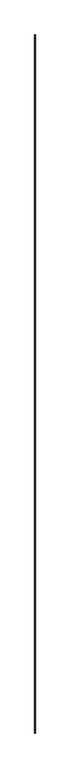
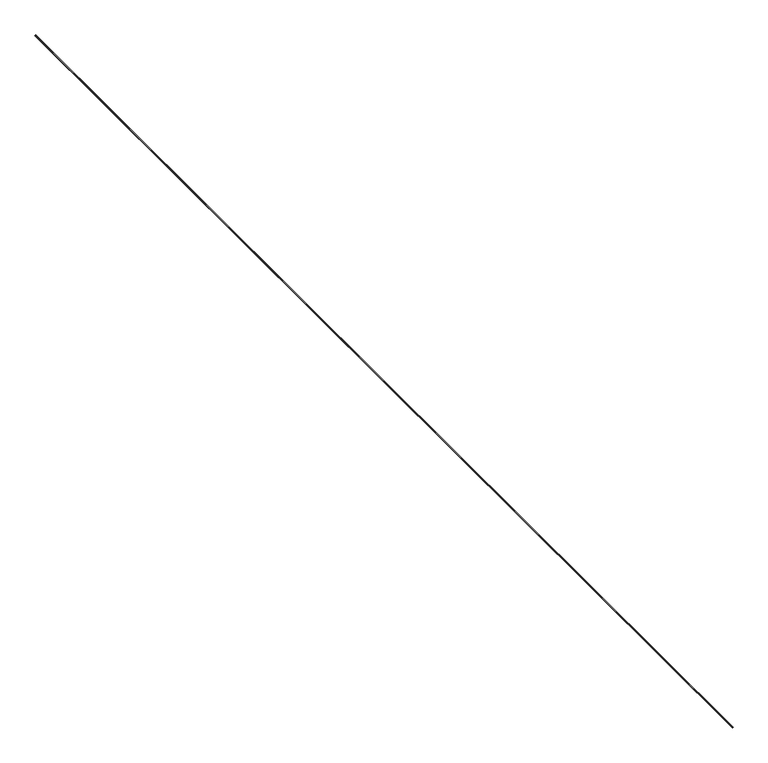
"""IFC4 building model written with IfcOpenShell, lengths in millimetres: proxy geometry, Inner panel:Inner panel:1:Inner panel:1 : Inner panel:Inner panel:300324:2:Inner panel:1:Inner panel:1 : Inner panel:Inner panel:300324:2 : Inner panel:Inner panel:1:Inner panel:1 : Inner panel:Inner panel:300324:300043:163 : Inner panel:Inner panel:1:Inner panel:1 : Inner panel:Inner panel:300324:2:Inner panel:1:Inner panel:1 : Inner panel:Inner panel:300324:2 : Inner panel:Inner panel:1:Inner panel:1 : Inner panel:Inner panel:300324:300043:308120."""

import ifcopenshell
import ifcopenshell.guid

model = None  # the IFC model being written
_history = None  # IfcOwnerHistory: only IFC2X3 demands one
_inside = {}  # id of a spatial element -> (the spatial element, [elements in it])
_under = {}  # id of a project, library or spatial element -> (it, [spatial elements below it])
_declared = {}  # id of a project -> (the project, [libraries it declares])
_typed = {}  # id of a type object -> (the type object, [elements of that type])
_made_of = {}  # id of a material, layer set ... -> (it, [elements and type objects made of it])


def new_model(schema):
    """Start an empty IFC model of exactly this schema.

    Asked for "IFC4X3", IfcOpenShell would pick the latest addendum, in which some entities
    have other attributes; the version numbers below select the first issue.
    IFC2X3 requires an IfcOwnerHistory on every rooted entity: one is made here for all.
    """
    global model, _history
    if schema == "IFC4X3":
        model = ifcopenshell.file(schema_version=(4, 3, 0, 0))
    else:
        model = ifcopenshell.file(schema=schema)
    _inside.clear()
    _under.clear()
    _declared.clear()
    _typed.clear()
    _made_of.clear()
    _history = None
    if model.schema == "IFC2X3":
        org = make("IfcOrganization", Name="unknown")
        user = make(
            "IfcPersonAndOrganization",
            ThePerson=make("IfcPerson", FamilyName="unknown"),
            TheOrganization=org,
        )
        app = make(
            "IfcApplication",
            ApplicationDeveloper=org,
            Version="unknown",
            ApplicationFullName="unknown",
            ApplicationIdentifier="unknown",
        )
        _history = make(
            "IfcOwnerHistory",
            OwningUser=user,
            OwningApplication=app,
            ChangeAction="ADDED",
            CreationDate=0,
        )
    return model


def make(cls, **values):
    """One entity of the class cls with the attributes given. An attribute that is None is left unset."""
    return model.create_entity(
        cls, **{name: value for name, value in values.items() if value is not None}
    )


def rooted(cls, **values):
    """An entity with a GlobalId (a new one), such as an element, a storey or a relation."""
    return make(cls, GlobalId=ifcopenshell.guid.new(), OwnerHistory=_history, **values)


def si_unit(unit_type, name, prefix=None):
    """IfcSIUnit, for example si_unit("LENGTHUNIT", "METRE", prefix="MILLI")."""
    return make("IfcSIUnit", UnitType=unit_type, Prefix=prefix, Name=name)


def assignment(units):
    """IfcUnitAssignment: the units of a project."""
    return None if units is None else make("IfcUnitAssignment", Units=units)


def point(xyz):
    """IfcCartesianPoint."""
    return None if xyz is None else make("IfcCartesianPoint", Coordinates=xyz)


def direction(xyz):
    """IfcDirection."""
    return None if xyz is None else make("IfcDirection", DirectionRatios=xyz)


def frame(location, z_axis=None, x_axis=None):
    """IfcAxis2Placement3D, a coordinate frame: its origin and axes. An axis left out is left unset."""
    return make(
        "IfcAxis2Placement3D",
        Location=point(location),
        Axis=direction(z_axis),
        RefDirection=direction(x_axis),
    )


def origin():
    """The frame at (0, 0, 0) with its axes left unset."""
    return frame((0.0, 0.0, 0.0))


def place(relative_to, where):
    """IfcLocalPlacement: puts the frame where relative to a parent placement (None: the world)."""
    return make(
        "IfcLocalPlacement", PlacementRelTo=relative_to, RelativePlacement=where
    )


def context(
    kind, dimensions, precision=None, world=None, true_north=None, identifier=None
):
    """IfcGeometricRepresentationContext, for example the 3D "Model" context."""
    return make(
        "IfcGeometricRepresentationContext",
        ContextIdentifier=identifier,
        ContextType=kind,
        CoordinateSpaceDimension=dimensions,
        Precision=precision,
        WorldCoordinateSystem=world,
        TrueNorth=true_north,
    )


def project(units=None, contexts=None):
    """IfcProject with its units and contexts."""
    return rooted(
        "IfcProject",
        Name="project",
        RepresentationContexts=contexts,
        UnitsInContext=assignment(units),
    )


def spatial(cls, under=None, at=None, **own):
    """A site, building, storey or space (cls), placed at a placement, below another one or the project."""
    s = rooted(cls, ObjectPlacement=at, **own)
    if under is not None:
        _under.setdefault(under.id(), (under, []))[1].append(s)
    return s


def polyline(points):
    """IfcPolyline through the points."""
    return make("IfcPolyline", Points=[point(p) for p in points])


def outline(outer, holes=None, kind="AREA"):
    """IfcArbitraryClosedProfileDef: a profile drawn as a closed curve; with holes, ...WithVoids."""
    if holes is None:
        return make("IfcArbitraryClosedProfileDef", ProfileType=kind, OuterCurve=outer)
    return make(
        "IfcArbitraryProfileDefWithVoids",
        ProfileType=kind,
        OuterCurve=outer,
        InnerCurves=holes,
    )


def extrude(swept, where, along, depth):
    """IfcExtrudedAreaSolid: the profile swept, set in the frame where, extruded along a direction by depth."""
    return make(
        "IfcExtrudedAreaSolid",
        SweptArea=swept,
        Position=where,
        ExtrudedDirection=direction(along),
        Depth=depth,
    )


def shape(context_of_items, identifier, shape_type, items):
    """IfcShapeRepresentation: the items that make up one representation, for example the "Body"."""
    return make(
        "IfcShapeRepresentation",
        ContextOfItems=context_of_items,
        RepresentationIdentifier=identifier,
        RepresentationType=shape_type,
        Items=items,
    )


def source(mapping_origin, context_of_items, identifier, shape_type, items):
    """IfcRepresentationMap: a shape defined once, which mapped items show again and again."""
    return make(
        "IfcRepresentationMap",
        MappingOrigin=mapping_origin,
        MappedRepresentation=shape(context_of_items, identifier, shape_type, items),
    )


def transform(
    local_origin,
    x_axis=None,
    y_axis=None,
    z_axis=None,
    scale=None,
    scale2=None,
    scale3=None,
    uniform=True,
):
    """IfcCartesianTransformationOperator3D, or its non-uniform kind. x_axis, y_axis, z_axis: its Axis1, 2, 3."""
    if uniform:
        return make(
            "IfcCartesianTransformationOperator3D",
            Axis1=direction(x_axis),
            Axis2=direction(y_axis),
            LocalOrigin=point(local_origin),
            Scale=scale,
            Axis3=direction(z_axis),
        )
    return make(
        "IfcCartesianTransformationOperator3DnonUniform",
        Axis1=direction(x_axis),
        Axis2=direction(y_axis),
        LocalOrigin=point(local_origin),
        Scale=scale,
        Axis3=direction(z_axis),
        Scale2=scale2,
        Scale3=scale3,
    )


def mapped(mapping_source, mapping_target):
    """IfcMappedItem: shows the shape of a source again, moved by a transform."""
    return make(
        "IfcMappedItem", MappingSource=mapping_source, MappingTarget=mapping_target
    )


def made_of(thing, what):
    """Note that an element or type object is made of a material, layer set ...; save() writes the relation."""
    if what is not None:
        _made_of.setdefault(what.id(), (what, []))[1].append(thing)
    return thing


def element(
    cls,
    number,
    at=None,
    inside=None,
    cuts=None,
    type_object=None,
    material=None,
    context=None,
    identifier="Body",
    shape_type=None,
    held_by="IfcProductDefinitionShape",
    body=None,
    shapes=None,
    **own,
):
    """One element of the class cls, such as IfcWall. Its Tag is "e" and its number.

    at: its placement. inside: the storey or other place that contains it. cuts: it is an
    opening in that element (IfcRelVoidsElement). A single representation is given by context,
    identifier, shape_type and body (its items); several are given by shapes. held_by: the class
    of the entity that holds the representations. save() writes the other relations.
    """
    e = rooted(cls, Tag="e%d" % number, ObjectPlacement=at, **own)
    if body is not None:
        shapes = [shape(context, identifier, shape_type, body)]
    if shapes is not None:
        e.Representation = make(held_by, Representations=shapes)
    if inside is not None:
        _inside.setdefault(inside.id(), (inside, []))[1].append(e)
    if cuts is not None:
        rooted(
            "IfcRelVoidsElement", RelatingBuildingElement=cuts, RelatedOpeningElement=e
        )
    if type_object is not None:
        _typed.setdefault(type_object.id(), (type_object, []))[1].append(e)
    return made_of(e, material)


def aggregate(whole, parts):
    """IfcRelAggregates: a whole, such as a stair, and the parts it consists of."""
    return rooted("IfcRelAggregates", RelatingObject=whole, RelatedObjects=parts)


def save(model, path):
    """Write the relations noted so far, then the file.

    IfcRelAggregates (storeys below a building ...), IfcRelContainedInSpatialStructure (elements
    in a storey), IfcRelDefinesByType, IfcRelAssociatesMaterial and IfcRelDeclares: one each for
    every whole, place, type object, material and project.
    """
    for whole, parts in _under.values():
        aggregate(whole, parts)
    for where, things in _inside.values():
        rooted(
            "IfcRelContainedInSpatialStructure",
            RelatedElements=things,
            RelatingStructure=where,
        )
    for kind, things in _typed.values():
        rooted("IfcRelDefinesByType", RelatedObjects=things, RelatingType=kind)
    for what, things in _made_of.values():
        rooted("IfcRelAssociatesMaterial", RelatedObjects=things, RelatingMaterial=what)
    for by, libraries in _declared.values():
        rooted("IfcRelDeclares", RelatingContext=by, RelatedDefinitions=libraries)
    model.write(path)


def generic_models_3eed4567(model_context):
    return source(origin(), model_context, "Body", "SweptSolid", [
        extrude(outline(polyline([(3912.8322781, 560391.2693699), (3913.5270451, 560407.9437769), (3917.2347295, 560407.7892901), (3917.2347295, 560406.2004127), (3915.0470803, 560406.2915647), (3914.4844903, 560392.7894052), (3950.9653367, 560391.26937), (3949.0465699, 560345.2189662), (3912.5657235, 560346.7390014), (3912.0031335, 560333.2368419), (3914.1246942, 560333.1484436), (3914.1246942, 560331.5595661), (3910.3509213, 560331.7168067), (3911.0456883, 560348.3912137), (3947.5265346, 560346.8711784), (3949.3131244, 560389.7493347), (3912.8322781, 560391.2693699)])), frame((0.0, -579013.3913841, 0.0), z_axis=(0.0, 1.0, 0.0), x_axis=(0.0, 0.0, 1.0)), (0.0, 0.0, 1.0), 88442.8),
    ])


if __name__ == "__main__":
    model = new_model("IFC4")
    model_context = context("Model", 3, world=origin())
    ifc_project = project(units=[si_unit("LENGTHUNIT", "METRE", prefix="MILLI")], contexts=[model_context])
    site = spatial("IfcSite", under=ifc_project)
    building = spatial("IfcBuilding", under=site)
    placement = place(None, origin())
    generic_models_shape = generic_models_3eed4567(model_context)
    element("IfcBuildingElementProxy", 1, Name="Inner panel:Inner panel:1:Inner panel:1 : Inner panel:Inner panel:300324:2:Inner panel:1:Inner panel:1 : Inner panel:Inner panel:300324:2 : Inner panel:Inner panel:1:Inner panel:1 : Inner panel:Inner panel:300324:300043:163 : Inner panel:Inner panel:1:Inner panel:1 : Inner panel:Inner panel:300324:2:Inner panel:1:Inner panel:1 : Inner panel:Inner panel:300324:2 : Inner panel:Inner panel:1:Inner panel:1 : Inner panel:Inner panel:300324:300043:308120", ObjectType="Inner panel:Inner panel:1:Inner panel:1 : Inner panel:Inner panel:300324:2:Inner panel:1:Inner panel:1 : Inner panel:Inner panel:300324:2 : Inner panel:Inner panel:1:Inner panel:1 : Inner panel:Inner panel:300324:300043:163 : Inner panel:Inner panel:1:Inner panel:1 : Inner panel:Inner panel:300324:2:Inner panel:1:Inner panel:1 : Inner panel:Inner panel:300324:2 : Inner panel:Inner panel:1:Inner panel:1 : Inner panel:Inner panel:300324:300043:308120", at=placement, inside=building, context=model_context, shape_type="MappedRepresentation", body=[
        mapped(generic_models_shape, transform((0.0, 0.0, 0.0), x_axis=(1.0, 0.0, 0.0), y_axis=(0.0, 1.0, 0.0), z_axis=(0.0, 0.0, 1.0))),
    ])
    save(model, "model.ifc")

# Revit data of these elements
# Type "Inner panel:Inner panel:1:Inner panel:1 : Inner panel:Inner panel:300324:2:Inner panel:1:Inner panel:1 : Inner panel:Inner panel:300324:2 : Inner panel:Inner panel:1:Inner panel:1 : Inner panel:Inner panel:300324:300043:163 : Inner panel:Inner panel:1:Inner panel:1 : Inner panel:Inner panel:300324:2:Inner panel:1:Inner panel:1 : Inner panel:Inner panel:300324:2 : Inner panel:Inner panel:1:Inner panel:1 : Inner panel:Inner panel:300324:300043:308120"
#   NameOverride = "Inner panel:Inner panel:1:Inner panel:1 : Inner panel:Inner panel:300324:2:Inner panel:1:Inner panel:1 : Inner panel:Inner panel:300324:2 : Inner panel:Inner panel:1:Inner panel:1 : Inner panel:Inner panel:300324:300043:308120"
#   ObjectTypeOverride = "Inner panel:1:Inner panel:1 : Inner panel:Inner panel:300324:2 : Inner panel:Inner panel:1:Inner panel:1 : Inner panel:Inner panel:300324:300043"
#   Reference = "Inner panel"
#   Tag = "308120"
# Element 1 (IfcBuildingElementProxy, "Inner panel:Inner panel:1:Inner panel:1 : Inner panel:Inner panel:300324:2:Inner panel:1:Inner panel:1 : Inner panel:Inner panel:300324:2 : Inner panel:Inner panel:1:Inner panel:1 : Inner panel:Inner panel:300324:300043:163 : Inner panel:Inner panel:1:Inner panel:1 : Inner panel:Inner panel:300324:2:Inner panel:1:Inner panel:1 : Inner panel:Inner panel:300324:2 : Inner panel:Inner panel:1:Inner panel:1 : Inner panel:Inner panel:300324:300043:308120")
#   Materials on its faces: "1 1/2\" HAT CHANNELS - SEE STRUCT. DWGs"
# Materials
#   "1 1/2\" HAT CHANNELS - SEE STRUCT. DWGs": class "Metal", colour RGB 189 187 185, transparency 0, Description = "Structural steel 50ksi", Cost = 0
